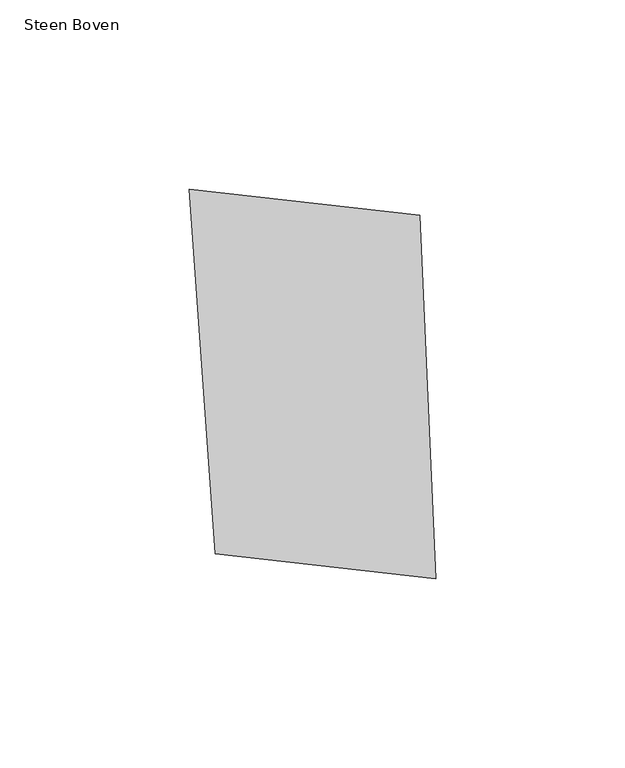
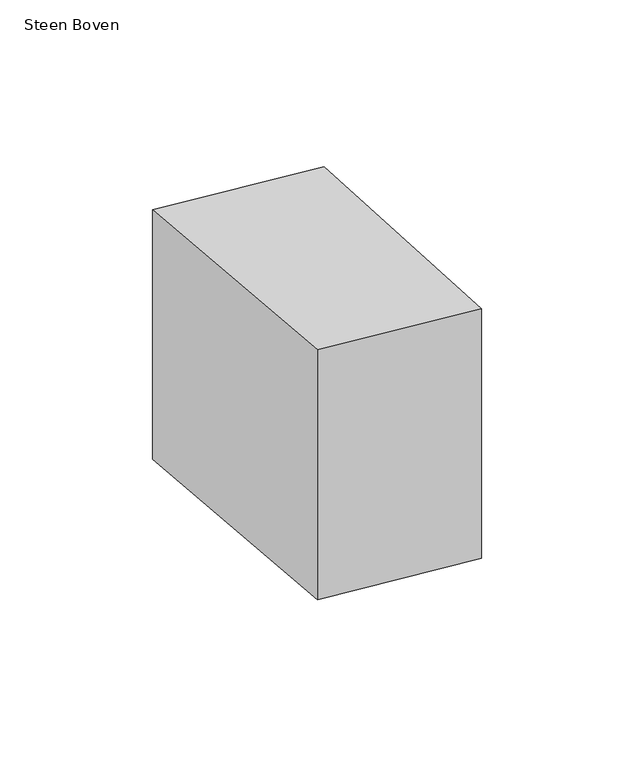
"""IFC4 building model written with IfcOpenShell, lengths in millimetres: proxy geometry, 00_GMA_steen_versie_4 : Steen Boven."""

from ifc_helpers import new_model, si_unit, origin, origin_with_axes, place, context, project, spatial, polyline, outline, extrude, source, transform, mapped, element, save


def steen_boven_65cc402e(model_context):
    return source(origin(), model_context, "Body", "SweptSolid", [
        extrude(outline(polyline([(98.3974268, 119.7245883), (102.5559242, 23.5856348), (44.2174986, 30.1644925), (37.3581209, 126.6291169), (98.3974268, 119.7245883)])), origin_with_axes(), (0.0, 0.0, 1.0), 100.0),
    ])


if __name__ == "__main__":
    model = new_model("IFC4")
    model_context = context("Model", 3, world=origin())
    ifc_project = project(units=[si_unit("LENGTHUNIT", "METRE", prefix="MILLI")], contexts=[model_context])
    site = spatial("IfcSite", under=ifc_project)
    building = spatial("IfcBuilding", under=site)
    placement = place(None, origin())
    steen_boven_shape = steen_boven_65cc402e(model_context)
    element("IfcBuildingElementProxy", 1, Name="00_GMA_steen_versie_4 : Steen Boven", ObjectType="00_GMA_steen_versie_4 : Steen Boven", at=placement, inside=building, context=model_context, shape_type="MappedRepresentation", body=[
        mapped(steen_boven_shape, transform((0.0, 0.0, 0.0), x_axis=(1.0, 0.0, 0.0), y_axis=(0.0, 1.0, 0.0), z_axis=(0.0, 0.0, 1.0))),
    ])
    save(model, "model.ifc")

# Revit data of these elements
# Type "00_GMA_steen_versie_4 : Steen Boven"
#   StootVoegHalfBoven [instance default] = 5 mm
#   StootVoegHalf [instance default] = 5 mm
#   StootVoegBreedteOnder = 10 mm
#   StootVoegBreedteBoven = 10 mm
#   Steendikte = 100 mm
#   LintVoegOnderHalf = 5 mm
#   LintVoegOnder = 10 mm
#   LintVoegBovenHalf = 0 mm
#   LintVoegBoven = 0 mm
#   materiaal = none
#   MateriaalVoeg = none
#   Default Elevation = 0
